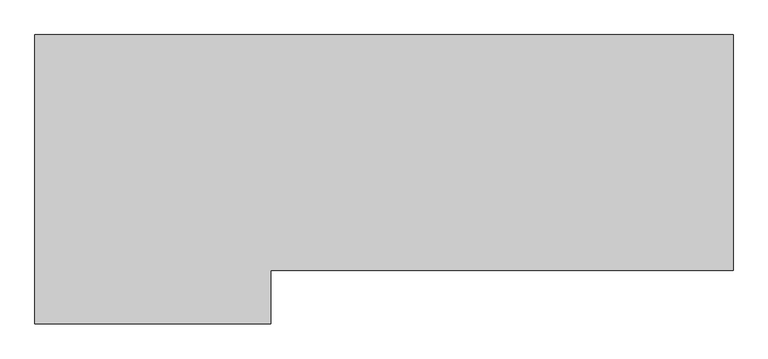
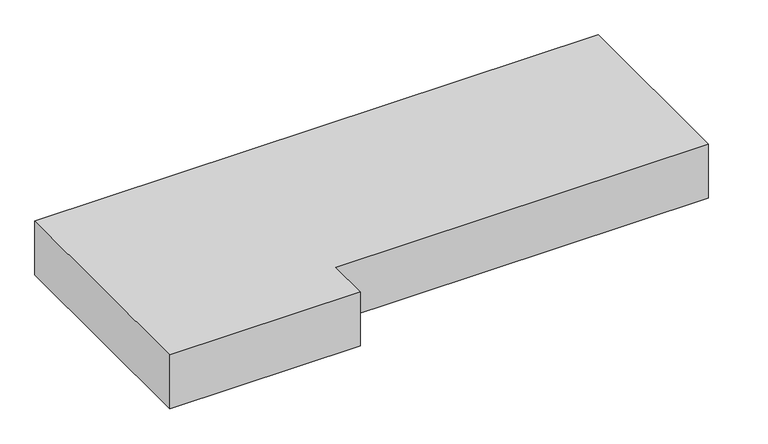
"""IFC4 building model written with IfcOpenShell, lengths in millimetres: proxy geometry, Deckendurchbruch."""

from ifc_helpers import new_model, si_unit, origin, origin_with_axes, place, context, project, spatial, polyline, outline, extrude, source, transform, mapped, element, save


def generic_models_29544a30(model_context):
    return source(origin(), model_context, "Body", "SweptSolid", [
        extrude(outline(polyline([(0.0, 1104.7357059), (2664.6018366, 1104.7357059), (2664.6018366, 204.7357059), (900.0, 204.7357059), (900.0, 0.0), (0.0, 0.0), (0.0, 1104.7357059)])), origin_with_axes(), (0.0, 0.0, 1.0), 270.0),
    ])


if __name__ == "__main__":
    model = new_model("IFC4")
    model_context = context("Model", 3, world=origin())
    ifc_project = project(units=[si_unit("LENGTHUNIT", "METRE", prefix="MILLI")], contexts=[model_context])
    site = spatial("IfcSite", under=ifc_project)
    building = spatial("IfcBuilding", under=site)
    placement = place(None, origin())
    generic_models_shape = generic_models_29544a30(model_context)
    element("IfcBuildingElementProxy", 1, Name="Deckendurchbruch", ObjectType="Deckendurchbruch", at=placement, inside=building, context=model_context, shape_type="MappedRepresentation", body=[
        mapped(generic_models_shape, transform((0.0, 0.0, 0.0), x_axis=(1.0, 0.0, 0.0), y_axis=(0.0, 1.0, 0.0), z_axis=(0.0, 0.0, 1.0))),
    ])
    save(model, "model.ifc")

# Revit data of these elements
# Element 1 (IfcBuildingElementProxy, "Deckendurchbruch")
#   Materials on its faces: "IfcOpeningElement"
# Materials
#   "IfcOpeningElement": class "Unassigned", colour RGB 255 165 0, transparency 0.75
